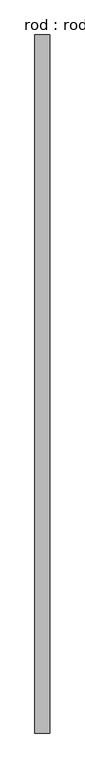
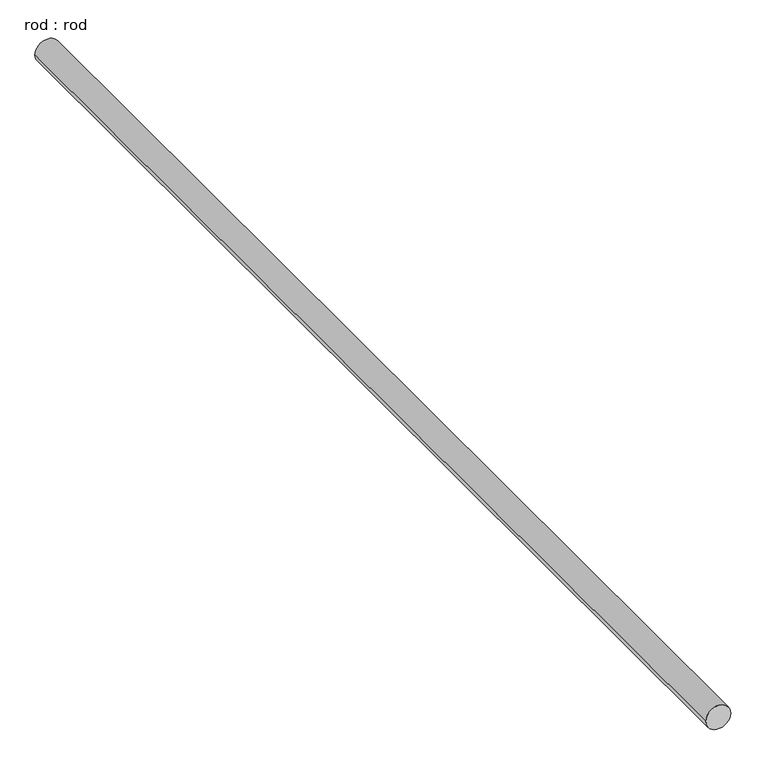
"""IFC4 building model written with IfcOpenShell, lengths in millimetres: proxy geometry, rod : rod."""

import ifcopenshell
import ifcopenshell.guid

model = None  # the IFC model being written
_history = None  # IfcOwnerHistory: only IFC2X3 demands one
_inside = {}  # id of a spatial element -> (the spatial element, [elements in it])
_under = {}  # id of a project, library or spatial element -> (it, [spatial elements below it])
_declared = {}  # id of a project -> (the project, [libraries it declares])
_typed = {}  # id of a type object -> (the type object, [elements of that type])
_made_of = {}  # id of a material, layer set ... -> (it, [elements and type objects made of it])


def new_model(schema):
    """Start an empty IFC model of exactly this schema.

    Asked for "IFC4X3", IfcOpenShell would pick the latest addendum, in which some entities
    have other attributes; the version numbers below select the first issue.
    IFC2X3 requires an IfcOwnerHistory on every rooted entity: one is made here for all.
    """
    global model, _history
    if schema == "IFC4X3":
        model = ifcopenshell.file(schema_version=(4, 3, 0, 0))
    else:
        model = ifcopenshell.file(schema=schema)
    _inside.clear()
    _under.clear()
    _declared.clear()
    _typed.clear()
    _made_of.clear()
    _history = None
    if model.schema == "IFC2X3":
        org = make("IfcOrganization", Name="unknown")
        user = make(
            "IfcPersonAndOrganization",
            ThePerson=make("IfcPerson", FamilyName="unknown"),
            TheOrganization=org,
        )
        app = make(
            "IfcApplication",
            ApplicationDeveloper=org,
            Version="unknown",
            ApplicationFullName="unknown",
            ApplicationIdentifier="unknown",
        )
        _history = make(
            "IfcOwnerHistory",
            OwningUser=user,
            OwningApplication=app,
            ChangeAction="ADDED",
            CreationDate=0,
        )
    return model


def make(cls, **values):
    """One entity of the class cls with the attributes given. An attribute that is None is left unset."""
    return model.create_entity(
        cls, **{name: value for name, value in values.items() if value is not None}
    )


def rooted(cls, **values):
    """An entity with a GlobalId (a new one), such as an element, a storey or a relation."""
    return make(cls, GlobalId=ifcopenshell.guid.new(), OwnerHistory=_history, **values)


def si_unit(unit_type, name, prefix=None):
    """IfcSIUnit, for example si_unit("LENGTHUNIT", "METRE", prefix="MILLI")."""
    return make("IfcSIUnit", UnitType=unit_type, Prefix=prefix, Name=name)


def assignment(units):
    """IfcUnitAssignment: the units of a project."""
    return None if units is None else make("IfcUnitAssignment", Units=units)


def point(xyz):
    """IfcCartesianPoint."""
    return None if xyz is None else make("IfcCartesianPoint", Coordinates=xyz)


def direction(xyz):
    """IfcDirection."""
    return None if xyz is None else make("IfcDirection", DirectionRatios=xyz)


def frame(location, z_axis=None, x_axis=None):
    """IfcAxis2Placement3D, a coordinate frame: its origin and axes. An axis left out is left unset."""
    return make(
        "IfcAxis2Placement3D",
        Location=point(location),
        Axis=direction(z_axis),
        RefDirection=direction(x_axis),
    )


def frame_2d(location, x_axis=None):
    """IfcAxis2Placement2D, a coordinate frame in the plane: its origin and x axis."""
    return make(
        "IfcAxis2Placement2D", Location=point(location), RefDirection=direction(x_axis)
    )


def origin():
    """The frame at (0, 0, 0) with its axes left unset."""
    return frame((0.0, 0.0, 0.0))


def place(relative_to, where):
    """IfcLocalPlacement: puts the frame where relative to a parent placement (None: the world)."""
    return make(
        "IfcLocalPlacement", PlacementRelTo=relative_to, RelativePlacement=where
    )


def context(
    kind, dimensions, precision=None, world=None, true_north=None, identifier=None
):
    """IfcGeometricRepresentationContext, for example the 3D "Model" context."""
    return make(
        "IfcGeometricRepresentationContext",
        ContextIdentifier=identifier,
        ContextType=kind,
        CoordinateSpaceDimension=dimensions,
        Precision=precision,
        WorldCoordinateSystem=world,
        TrueNorth=true_north,
    )


def project(units=None, contexts=None):
    """IfcProject with its units and contexts."""
    return rooted(
        "IfcProject",
        Name="project",
        RepresentationContexts=contexts,
        UnitsInContext=assignment(units),
    )


def spatial(cls, under=None, at=None, **own):
    """A site, building, storey or space (cls), placed at a placement, below another one or the project."""
    s = rooted(cls, ObjectPlacement=at, **own)
    if under is not None:
        _under.setdefault(under.id(), (under, []))[1].append(s)
    return s


def circle_curve(where, radius):
    """IfcCircle in the frame where."""
    return make("IfcCircle", Position=where, Radius=radius)


def trimmed(basis, trim1, trim2, sense, master):
    """IfcTrimmedCurve: the piece of a basis curve between two trims."""
    return make(
        "IfcTrimmedCurve",
        BasisCurve=basis,
        Trim1=trim1,
        Trim2=trim2,
        SenseAgreement=sense,
        MasterRepresentation=master,
    )


def segment(curve, same_sense, transition):
    """IfcCompositeCurveSegment."""
    return make(
        "IfcCompositeCurveSegment",
        Transition=transition,
        SameSense=same_sense,
        ParentCurve=curve,
    )


def composite_curve(segments, self_intersect=None):
    """IfcCompositeCurve: segments joined end to end."""
    return make("IfcCompositeCurve", Segments=segments, SelfIntersect=self_intersect)


def outline(outer, holes=None, kind="AREA"):
    """IfcArbitraryClosedProfileDef: a profile drawn as a closed curve; with holes, ...WithVoids."""
    if holes is None:
        return make("IfcArbitraryClosedProfileDef", ProfileType=kind, OuterCurve=outer)
    return make(
        "IfcArbitraryProfileDefWithVoids",
        ProfileType=kind,
        OuterCurve=outer,
        InnerCurves=holes,
    )


def extrude(swept, where, along, depth):
    """IfcExtrudedAreaSolid: the profile swept, set in the frame where, extruded along a direction by depth."""
    return make(
        "IfcExtrudedAreaSolid",
        SweptArea=swept,
        Position=where,
        ExtrudedDirection=direction(along),
        Depth=depth,
    )


def shape(context_of_items, identifier, shape_type, items):
    """IfcShapeRepresentation: the items that make up one representation, for example the "Body"."""
    return make(
        "IfcShapeRepresentation",
        ContextOfItems=context_of_items,
        RepresentationIdentifier=identifier,
        RepresentationType=shape_type,
        Items=items,
    )


def source(mapping_origin, context_of_items, identifier, shape_type, items):
    """IfcRepresentationMap: a shape defined once, which mapped items show again and again."""
    return make(
        "IfcRepresentationMap",
        MappingOrigin=mapping_origin,
        MappedRepresentation=shape(context_of_items, identifier, shape_type, items),
    )


def transform(
    local_origin,
    x_axis=None,
    y_axis=None,
    z_axis=None,
    scale=None,
    scale2=None,
    scale3=None,
    uniform=True,
):
    """IfcCartesianTransformationOperator3D, or its non-uniform kind. x_axis, y_axis, z_axis: its Axis1, 2, 3."""
    if uniform:
        return make(
            "IfcCartesianTransformationOperator3D",
            Axis1=direction(x_axis),
            Axis2=direction(y_axis),
            LocalOrigin=point(local_origin),
            Scale=scale,
            Axis3=direction(z_axis),
        )
    return make(
        "IfcCartesianTransformationOperator3DnonUniform",
        Axis1=direction(x_axis),
        Axis2=direction(y_axis),
        LocalOrigin=point(local_origin),
        Scale=scale,
        Axis3=direction(z_axis),
        Scale2=scale2,
        Scale3=scale3,
    )


def mapped(mapping_source, mapping_target):
    """IfcMappedItem: shows the shape of a source again, moved by a transform."""
    return make(
        "IfcMappedItem", MappingSource=mapping_source, MappingTarget=mapping_target
    )


def made_of(thing, what):
    """Note that an element or type object is made of a material, layer set ...; save() writes the relation."""
    if what is not None:
        _made_of.setdefault(what.id(), (what, []))[1].append(thing)
    return thing


def element(
    cls,
    number,
    at=None,
    inside=None,
    cuts=None,
    type_object=None,
    material=None,
    context=None,
    identifier="Body",
    shape_type=None,
    held_by="IfcProductDefinitionShape",
    body=None,
    shapes=None,
    **own,
):
    """One element of the class cls, such as IfcWall. Its Tag is "e" and its number.

    at: its placement. inside: the storey or other place that contains it. cuts: it is an
    opening in that element (IfcRelVoidsElement). A single representation is given by context,
    identifier, shape_type and body (its items); several are given by shapes. held_by: the class
    of the entity that holds the representations. save() writes the other relations.
    """
    e = rooted(cls, Tag="e%d" % number, ObjectPlacement=at, **own)
    if body is not None:
        shapes = [shape(context, identifier, shape_type, body)]
    if shapes is not None:
        e.Representation = make(held_by, Representations=shapes)
    if inside is not None:
        _inside.setdefault(inside.id(), (inside, []))[1].append(e)
    if cuts is not None:
        rooted(
            "IfcRelVoidsElement", RelatingBuildingElement=cuts, RelatedOpeningElement=e
        )
    if type_object is not None:
        _typed.setdefault(type_object.id(), (type_object, []))[1].append(e)
    return made_of(e, material)


def aggregate(whole, parts):
    """IfcRelAggregates: a whole, such as a stair, and the parts it consists of."""
    return rooted("IfcRelAggregates", RelatingObject=whole, RelatedObjects=parts)


def save(model, path):
    """Write the relations noted so far, then the file.

    IfcRelAggregates (storeys below a building ...), IfcRelContainedInSpatialStructure (elements
    in a storey), IfcRelDefinesByType, IfcRelAssociatesMaterial and IfcRelDeclares: one each for
    every whole, place, type object, material and project.
    """
    for whole, parts in _under.values():
        aggregate(whole, parts)
    for where, things in _inside.values():
        rooted(
            "IfcRelContainedInSpatialStructure",
            RelatedElements=things,
            RelatingStructure=where,
        )
    for kind, things in _typed.values():
        rooted("IfcRelDefinesByType", RelatedObjects=things, RelatingType=kind)
    for what, things in _made_of.values():
        rooted("IfcRelAssociatesMaterial", RelatedObjects=things, RelatingMaterial=what)
    for by, libraries in _declared.values():
        rooted("IfcRelDeclares", RelatingContext=by, RelatedDefinitions=libraries)
    model.write(path)


def rod_rod_f5e0b0fd(model_context):
    return source(origin(), model_context, "Body", "SweptSolid", [
        extrude(outline(composite_curve([segment(trimmed(circle_curve(frame_2d((0.0108462, 0.0)), 200.0), [point((0.0108462, 200.0))], [point((0.0108462, -200.0))], False, "CARTESIAN"), True, "CONTINUOUS"), segment(trimmed(circle_curve(frame_2d((0.0108462, 0.0)), 200.0), [point((0.0108462, -200.0))], [point((0.0108462, 200.0))], False, "CARTESIAN"), True, "CONTINUOUS")], self_intersect=False)), frame((0.0, -5268.8785275, 0.0), z_axis=(0.0, 1.0, 0.0), x_axis=(0.0, 0.0, 1.0)), (0.0, 0.0, 1.0), 18723.2142857),
    ])


if __name__ == "__main__":
    model = new_model("IFC4")
    model_context = context("Model", 3, world=origin())
    ifc_project = project(units=[si_unit("LENGTHUNIT", "METRE", prefix="MILLI")], contexts=[model_context])
    site = spatial("IfcSite", under=ifc_project)
    building = spatial("IfcBuilding", under=site)
    placement = place(None, origin())
    rod_rod_shape = rod_rod_f5e0b0fd(model_context)
    element("IfcBuildingElementProxy", 1, Name="rod : rod", ObjectType="rod : rod", at=placement, inside=building, context=model_context, shape_type="MappedRepresentation", body=[
        mapped(rod_rod_shape, transform((0.0, 0.0, 0.0), x_axis=(1.0, 0.0, 0.0), y_axis=(0.0, 1.0, 0.0), z_axis=(0.0, 0.0, 1.0))),
    ])
    save(model, "model.ifc")

# Revit data of these elements
# Type "rod : rod"
#   Default Elevation = 0
